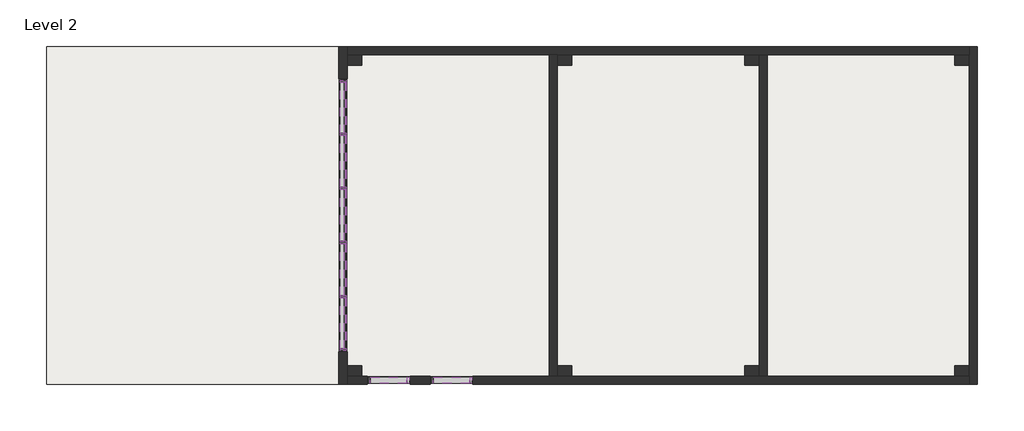
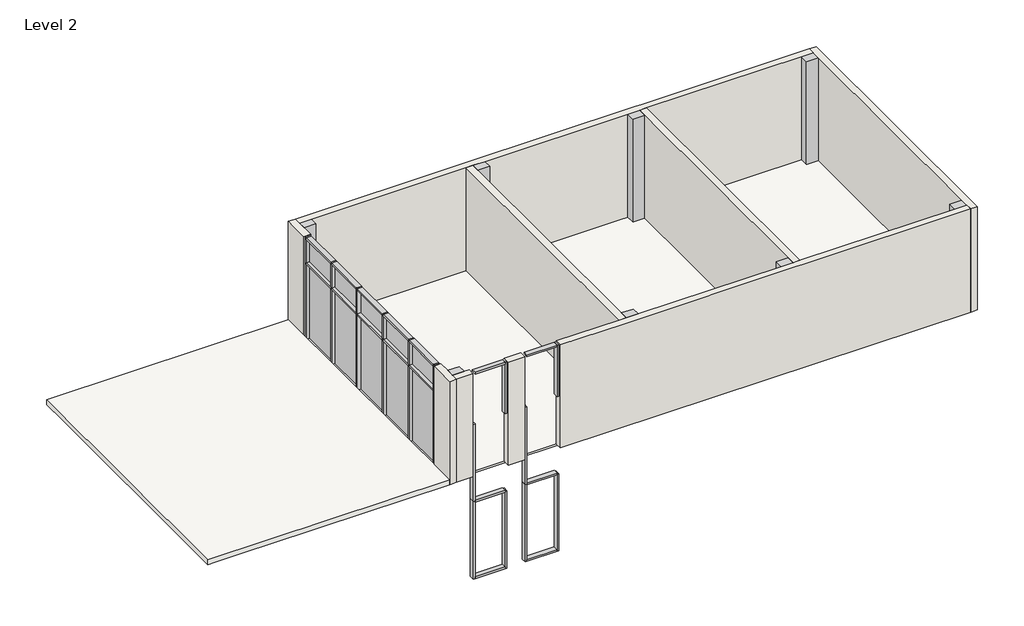
# One storey: 41 members, 10 plates, 9 walls, 8 columns, 3 slabs, 1 roof.
"""IFC4 building model written with IfcOpenShell, lengths in millimetres."""

import ifcopenshell
import ifcopenshell.guid

model = None  # the IFC model being written
_history = None  # IfcOwnerHistory: only IFC2X3 demands one
_inside = {}  # id of a spatial element -> (the spatial element, [elements in it])
_under = {}  # id of a project, library or spatial element -> (it, [spatial elements below it])
_declared = {}  # id of a project -> (the project, [libraries it declares])
_typed = {}  # id of a type object -> (the type object, [elements of that type])
_made_of = {}  # id of a material, layer set ... -> (it, [elements and type objects made of it])


def new_model(schema):
    """Start an empty IFC model of exactly this schema.

    Asked for "IFC4X3", IfcOpenShell would pick the latest addendum, in which some entities
    have other attributes; the version numbers below select the first issue.
    IFC2X3 requires an IfcOwnerHistory on every rooted entity: one is made here for all.
    """
    global model, _history
    if schema == "IFC4X3":
        model = ifcopenshell.file(schema_version=(4, 3, 0, 0))
    else:
        model = ifcopenshell.file(schema=schema)
    _inside.clear()
    _under.clear()
    _declared.clear()
    _typed.clear()
    _made_of.clear()
    _history = None
    if model.schema == "IFC2X3":
        org = make("IfcOrganization", Name="unknown")
        user = make(
            "IfcPersonAndOrganization",
            ThePerson=make("IfcPerson", FamilyName="unknown"),
            TheOrganization=org,
        )
        app = make(
            "IfcApplication",
            ApplicationDeveloper=org,
            Version="unknown",
            ApplicationFullName="unknown",
            ApplicationIdentifier="unknown",
        )
        _history = make(
            "IfcOwnerHistory",
            OwningUser=user,
            OwningApplication=app,
            ChangeAction="ADDED",
            CreationDate=0,
        )
    return model


def make(cls, **values):
    """One entity of the class cls with the attributes given. An attribute that is None is left unset."""
    return model.create_entity(
        cls, **{name: value for name, value in values.items() if value is not None}
    )


def rooted(cls, **values):
    """An entity with a GlobalId (a new one), such as an element, a storey or a relation."""
    return make(cls, GlobalId=ifcopenshell.guid.new(), OwnerHistory=_history, **values)


def si_unit(unit_type, name, prefix=None):
    """IfcSIUnit, for example si_unit("LENGTHUNIT", "METRE", prefix="MILLI")."""
    return make("IfcSIUnit", UnitType=unit_type, Prefix=prefix, Name=name)


def assignment(units):
    """IfcUnitAssignment: the units of a project."""
    return None if units is None else make("IfcUnitAssignment", Units=units)


def point(xyz):
    """IfcCartesianPoint."""
    return None if xyz is None else make("IfcCartesianPoint", Coordinates=xyz)


def direction(xyz):
    """IfcDirection."""
    return None if xyz is None else make("IfcDirection", DirectionRatios=xyz)


def frame(location, z_axis=None, x_axis=None):
    """IfcAxis2Placement3D, a coordinate frame: its origin and axes. An axis left out is left unset."""
    return make(
        "IfcAxis2Placement3D",
        Location=point(location),
        Axis=direction(z_axis),
        RefDirection=direction(x_axis),
    )


def origin():
    """The frame at (0, 0, 0) with its axes left unset."""
    return frame((0.0, 0.0, 0.0))


def origin_with_axes():
    """The frame at (0, 0, 0) with the z axis (0, 0, 1) and the x axis (1, 0, 0) written out."""
    return frame((0.0, 0.0, 0.0), z_axis=(0.0, 0.0, 1.0), x_axis=(1.0, 0.0, 0.0))


def place(relative_to, where):
    """IfcLocalPlacement: puts the frame where relative to a parent placement (None: the world)."""
    return make(
        "IfcLocalPlacement", PlacementRelTo=relative_to, RelativePlacement=where
    )


def context(
    kind, dimensions, precision=None, world=None, true_north=None, identifier=None
):
    """IfcGeometricRepresentationContext, for example the 3D "Model" context."""
    return make(
        "IfcGeometricRepresentationContext",
        ContextIdentifier=identifier,
        ContextType=kind,
        CoordinateSpaceDimension=dimensions,
        Precision=precision,
        WorldCoordinateSystem=world,
        TrueNorth=true_north,
    )


def project(units=None, contexts=None):
    """IfcProject with its units and contexts."""
    return rooted(
        "IfcProject",
        Name="project",
        RepresentationContexts=contexts,
        UnitsInContext=assignment(units),
    )


def spatial(cls, under=None, at=None, **own):
    """A site, building, storey or space (cls), placed at a placement, below another one or the project."""
    s = rooted(cls, ObjectPlacement=at, **own)
    if under is not None:
        _under.setdefault(under.id(), (under, []))[1].append(s)
    return s


def polyline(points):
    """IfcPolyline through the points."""
    return make("IfcPolyline", Points=[point(p) for p in points])


def outline(outer, holes=None, kind="AREA"):
    """IfcArbitraryClosedProfileDef: a profile drawn as a closed curve; with holes, ...WithVoids."""
    if holes is None:
        return make("IfcArbitraryClosedProfileDef", ProfileType=kind, OuterCurve=outer)
    return make(
        "IfcArbitraryProfileDefWithVoids",
        ProfileType=kind,
        OuterCurve=outer,
        InnerCurves=holes,
    )


def extrude(swept, where, along, depth):
    """IfcExtrudedAreaSolid: the profile swept, set in the frame where, extruded along a direction by depth."""
    return make(
        "IfcExtrudedAreaSolid",
        SweptArea=swept,
        Position=where,
        ExtrudedDirection=direction(along),
        Depth=depth,
    )


def faces_of(points, faces, orient=None, outer=None):
    """IfcFace entities. A face is a list of loops; a loop is a list of indices into points, from 0.

    orient and outer hold one flag for each loop. By default every Orientation is true, the
    first loop of a face is its IfcFaceOuterBound and the others are IfcFaceBound.
    """
    made = []
    for i, loops in enumerate(faces):
        bounds = []
        for j, loop in enumerate(loops):
            is_outer = j == 0 if outer is None else outer[i][j]
            bounds.append(
                make(
                    "IfcFaceOuterBound" if is_outer else "IfcFaceBound",
                    Bound=make("IfcPolyLoop", Polygon=[points[k] for k in loop]),
                    Orientation=True if orient is None else orient[i][j],
                )
            )
        made.append(make("IfcFace", Bounds=bounds))
    return made


def faceted_brep(points, faces, orient=None, outer=None, voids=None):
    """IfcFacetedBrep: a solid bounded by flat faces; with voids (closed shells), ...WithVoids."""
    shared = [point(p) for p in points]
    hull = make("IfcClosedShell", CfsFaces=faces_of(shared, faces, orient, outer))
    if voids is None:
        return make("IfcFacetedBrep", Outer=hull)
    return make(
        "IfcFacetedBrepWithVoids",
        Outer=hull,
        Voids=[
            make(cls, CfsFaces=faces_of(shared, fs, o, b)) for cls, fs, o, b in voids
        ],
    )


def shape(context_of_items, identifier, shape_type, items):
    """IfcShapeRepresentation: the items that make up one representation, for example the "Body"."""
    return make(
        "IfcShapeRepresentation",
        ContextOfItems=context_of_items,
        RepresentationIdentifier=identifier,
        RepresentationType=shape_type,
        Items=items,
    )


def source(mapping_origin, context_of_items, identifier, shape_type, items):
    """IfcRepresentationMap: a shape defined once, which mapped items show again and again."""
    return make(
        "IfcRepresentationMap",
        MappingOrigin=mapping_origin,
        MappedRepresentation=shape(context_of_items, identifier, shape_type, items),
    )


def transform(
    local_origin,
    x_axis=None,
    y_axis=None,
    z_axis=None,
    scale=None,
    scale2=None,
    scale3=None,
    uniform=True,
):
    """IfcCartesianTransformationOperator3D, or its non-uniform kind. x_axis, y_axis, z_axis: its Axis1, 2, 3."""
    if uniform:
        return make(
            "IfcCartesianTransformationOperator3D",
            Axis1=direction(x_axis),
            Axis2=direction(y_axis),
            LocalOrigin=point(local_origin),
            Scale=scale,
            Axis3=direction(z_axis),
        )
    return make(
        "IfcCartesianTransformationOperator3DnonUniform",
        Axis1=direction(x_axis),
        Axis2=direction(y_axis),
        LocalOrigin=point(local_origin),
        Scale=scale,
        Axis3=direction(z_axis),
        Scale2=scale2,
        Scale3=scale3,
    )


def mapped(mapping_source, mapping_target):
    """IfcMappedItem: shows the shape of a source again, moved by a transform."""
    return make(
        "IfcMappedItem", MappingSource=mapping_source, MappingTarget=mapping_target
    )


def made_of(thing, what):
    """Note that an element or type object is made of a material, layer set ...; save() writes the relation."""
    if what is not None:
        _made_of.setdefault(what.id(), (what, []))[1].append(thing)
    return thing


def element(
    cls,
    number,
    at=None,
    inside=None,
    cuts=None,
    type_object=None,
    material=None,
    context=None,
    identifier="Body",
    shape_type=None,
    held_by="IfcProductDefinitionShape",
    body=None,
    shapes=None,
    **own,
):
    """One element of the class cls, such as IfcWall. Its Tag is "e" and its number.

    at: its placement. inside: the storey or other place that contains it. cuts: it is an
    opening in that element (IfcRelVoidsElement). A single representation is given by context,
    identifier, shape_type and body (its items); several are given by shapes. held_by: the class
    of the entity that holds the representations. save() writes the other relations.
    """
    e = rooted(cls, Tag="e%d" % number, ObjectPlacement=at, **own)
    if body is not None:
        shapes = [shape(context, identifier, shape_type, body)]
    if shapes is not None:
        e.Representation = make(held_by, Representations=shapes)
    if inside is not None:
        _inside.setdefault(inside.id(), (inside, []))[1].append(e)
    if cuts is not None:
        rooted(
            "IfcRelVoidsElement", RelatingBuildingElement=cuts, RelatedOpeningElement=e
        )
    if type_object is not None:
        _typed.setdefault(type_object.id(), (type_object, []))[1].append(e)
    return made_of(e, material)


def aggregate(whole, parts):
    """IfcRelAggregates: a whole, such as a stair, and the parts it consists of."""
    return rooted("IfcRelAggregates", RelatingObject=whole, RelatedObjects=parts)


def save(model, path):
    """Write the relations noted so far, then the file.

    IfcRelAggregates (storeys below a building ...), IfcRelContainedInSpatialStructure (elements
    in a storey), IfcRelDefinesByType, IfcRelAssociatesMaterial and IfcRelDeclares: one each for
    every whole, place, type object, material and project.
    """
    for whole, parts in _under.values():
        aggregate(whole, parts)
    for where, things in _inside.values():
        rooted(
            "IfcRelContainedInSpatialStructure",
            RelatedElements=things,
            RelatingStructure=where,
        )
    for kind, things in _typed.values():
        rooted("IfcRelDefinesByType", RelatedObjects=things, RelatingType=kind)
    for what, things in _made_of.values():
        rooted("IfcRelAssociatesMaterial", RelatedObjects=things, RelatingMaterial=what)
    for by, libraries in _declared.values():
        rooted("IfcRelDeclares", RelatingContext=by, RelatedDefinitions=libraries)
    model.write(path)


def rectangular_mullion_50_x_150mm_49395e3f(model_context):
    return source(origin(), model_context, "Body", "SweptSolid", [
        extrude(outline(polyline([(0.0, 75.0), (0.0, -75.0), (-50.0, -75.0), (-50.0, 75.0), (0.0, 75.0)])), frame((0.0, 0.0, -1240.0000002), z_axis=(0.0, 0.0, 1.0), x_axis=(1.0, 0.0, 0.0)), (0.0, 0.0, 1.0), 1240.0000002),
    ])


def rectangular_mullion_50_x_150mm_673792d4(model_context):
    return source(origin(), model_context, "Body", "SweptSolid", [
        extrude(outline(polyline([(0.0, 75.0), (0.0, -75.0), (-50.0, -75.0), (-50.0, 75.0), (0.0, 75.0)])), frame((0.0, 0.0, -1264.9999999), z_axis=(0.0, 0.0, 1.0), x_axis=(1.0, 0.0, 0.0)), (0.0, 0.0, 1.0), 1264.9999999),
    ])


def rectangular_mullion_50_x_150mm_23e890aa(model_context):
    return source(origin(), model_context, "Body", "SweptSolid", [
        extrude(outline(polyline([(25.0, 75.0), (25.0, -75.0), (-25.0, -75.0), (-25.0, 75.0), (25.0, 75.0)])), frame((0.0, 0.0, -1240.0000002), z_axis=(0.0, 0.0, 1.0), x_axis=(1.0, 0.0, 0.0)), (0.0, 0.0, 1.0), 1240.0000002),
    ])


def rectangular_mullion_50_x_150mm_97c2790d(model_context):
    return source(origin(), model_context, "Body", "SweptSolid", [
        extrude(outline(polyline([(25.0, 75.0), (25.0, -75.0), (-25.0, -75.0), (-25.0, 75.0), (25.0, 75.0)])), frame((0.0, 0.0, -1264.9999999), z_axis=(0.0, 0.0, 1.0), x_axis=(1.0, 0.0, 0.0)), (0.0, 0.0, 1.0), 1264.9999999),
    ])


def rectangular_mullion_50_x_150mm_6225e4e3(model_context):
    return source(origin(), model_context, "Body", "SweptSolid", [
        extrude(outline(polyline([(25.0, 75.0), (25.0, -75.0), (-25.0, -75.0), (-25.0, 75.0), (25.0, 75.0)])), frame((0.0, 0.0, -2400.0), z_axis=(0.0, 0.0, 1.0), x_axis=(1.0, 0.0, 0.0)), (0.0, 0.0, 1.0), 2400.0),
    ])


def rectangular_mullion_50_x_150mm_14f10ac7(model_context):
    return source(origin(), model_context, "Body", "SweptSolid", [
        extrude(outline(polyline([(25.0, 75.0), (25.0, -75.0), (-25.0, -75.0), (-25.0, 75.0), (25.0, 75.0)])), frame((0.0, 0.0, -800.0), z_axis=(0.0, 0.0, 1.0), x_axis=(1.0, 0.0, 0.0)), (0.0, 0.0, 1.0), 800.0),
    ])


def rectangular_mullion_50_x_150mm_662c37b1(model_context):
    return source(origin(), model_context, "Body", "SweptSolid", [
        extrude(outline(polyline([(0.0, 75.0), (0.0, -75.0), (-50.0, -75.0), (-50.0, 75.0), (0.0, 75.0)])), frame((0.0, 0.0, -2400.0), z_axis=(0.0, 0.0, 1.0), x_axis=(1.0, 0.0, 0.0)), (0.0, 0.0, 1.0), 2400.0),
    ])


def rectangular_mullion_50_x_150mm_6ffebc0f(model_context):
    return source(origin(), model_context, "Body", "SweptSolid", [
        extrude(outline(polyline([(0.0, 75.0), (0.0, -75.0), (-50.0, -75.0), (-50.0, 75.0), (0.0, 75.0)])), frame((0.0, 0.0, -800.0), z_axis=(0.0, 0.0, 1.0), x_axis=(1.0, 0.0, 0.0)), (0.0, 0.0, 1.0), 800.0),
    ])


def rectangular_mullion_50_x_150mm_8ee200a5(model_context):
    return source(origin(), model_context, "Body", "SweptSolid", [
        extrude(outline(polyline([(0.0, 75.0), (0.0, -75.0), (-50.0, -75.0), (-50.0, 75.0), (0.0, 75.0)])), frame((0.0, 0.0, -887.5), z_axis=(0.0, 0.0, 1.0), x_axis=(1.0, 0.0, 0.0)), (0.0, 0.0, 1.0), 887.5),
    ])


def rectangular_mullion_50_x_150mm_6e645c27(model_context):
    return source(origin(), model_context, "Body", "SweptSolid", [
        extrude(outline(polyline([(25.0, 75.0), (25.0, -75.0), (-25.0, -75.0), (-25.0, 75.0), (25.0, 75.0)])), frame((0.0, 0.0, -887.5), z_axis=(0.0, 0.0, 1.0), x_axis=(1.0, 0.0, 0.0)), (0.0, 0.0, 1.0), 887.5),
    ])


def rectangular_mullion_50_x_150mm_849620c7(model_context):
    return source(origin(), model_context, "Body", "SweptSolid", [
        extrude(outline(polyline([(0.0, 75.0), (0.0, -75.0), (-50.0, -75.0), (-50.0, 75.0), (0.0, 75.0)])), frame((0.0, 0.0, -1600.0), z_axis=(0.0, 0.0, 1.0), x_axis=(1.0, 0.0, 0.0)), (0.0, 0.0, 1.0), 1600.0),
    ])


def system_panel_glazed_da598795(model_context):
    return source(origin(), model_context, "Body", "SweptSolid", [
        extrude(outline(polyline([(620.0000001, 24.5), (-620.0000001, 24.5), (-620.0000001, 49.5), (620.0000001, 49.5), (620.0000001, 24.5)])), origin_with_axes(), (0.0, 0.0, 1.0), 2325.0),
    ])


def system_panel_glazed_e4649fa4(model_context):
    return source(origin(), model_context, "Body", "SweptSolid", [
        extrude(outline(polyline([(632.4999999, 24.5), (-632.4999999, 24.5), (-632.4999999, 49.5), (632.4999999, 49.5), (632.4999999, 24.5)])), origin_with_axes(), (0.0, 0.0, 1.0), 2325.0),
    ])


def system_panel_glazed_8692f37a(model_context):
    return source(origin(), model_context, "Body", "SweptSolid", [
        extrude(outline(polyline([(620.0000001, 24.5), (-620.0000001, 24.5), (-620.0000001, 49.5), (620.0000001, 49.5), (620.0000001, 24.5)])), origin_with_axes(), (0.0, 0.0, 1.0), 725.0),
    ])


def system_panel_glazed_8e5047c4(model_context):
    return source(origin(), model_context, "Body", "SweptSolid", [
        extrude(outline(polyline([(632.4999999, 24.5), (-632.4999999, 24.5), (-632.4999999, 49.5), (632.4999999, 49.5), (632.4999999, 24.5)])), origin_with_axes(), (0.0, 0.0, 1.0), 725.0),
    ])


model = new_model("IFC4")

# Units and contexts
model_context = context("Model", 3, world=origin())
ifc_project = project(units=[si_unit("LENGTHUNIT", "METRE", prefix="MILLI")], contexts=[model_context])

# Site, building, storey
site = spatial("IfcSite", under=ifc_project)
building = spatial("IfcBuilding", under=site)
storey = spatial("IfcBuildingStorey", under=building, Name="Level 2", Elevation=3200.0)

# Columns
placement = place(None, origin())
element("IfcColumn", 1, ObjectType="M_Rectangular Column : 350 X 250", at=placement, inside=storey, context=model_context, shape_type="SweptSolid", body=[
    extrude(outline(polyline([(4723.8381324, 10606.2894154), (5073.8381324, 10606.2894154), (5073.8381324, 10356.2894154), (4723.8381324, 10356.2894154), (4723.8381324, 10606.2894154)])), frame((0.0, 0.0, 3200.0), z_axis=(0.0, 0.0, 1.0), x_axis=(1.0, 0.0, 0.0)), (0.0, 0.0, 1.0), 3200.0),
])
element("IfcColumn", 2, ObjectType="M_Rectangular Column : 350 X 250", at=placement, inside=storey, context=model_context, shape_type="SweptSolid", body=[
    extrude(outline(polyline([(4723.8381324, 3056.2894154), (5073.8381324, 3056.2894154), (5073.8381324, 2806.2894154), (4723.8381324, 2806.2894154), (4723.8381324, 3056.2894154)])), frame((0.0, 0.0, 3200.0), z_axis=(0.0, 0.0, 1.0), x_axis=(1.0, 0.0, 0.0)), (0.0, 0.0, 1.0), 3200.0),
])
element("IfcColumn", 3, ObjectType="M_Rectangular Column : 350 X 250", at=placement, inside=storey, context=model_context, shape_type="SweptSolid", body=[
    extrude(outline(polyline([(-376.1618676, 3056.2894154), (-26.1618676, 3056.2894154), (-26.1618676, 2806.2894154), (-376.1618676, 2806.2894154), (-376.1618676, 3056.2894154)])), frame((0.0, 0.0, 3200.0), z_axis=(0.0, 0.0, 1.0), x_axis=(1.0, 0.0, 0.0)), (0.0, 0.0, 1.0), 3200.0),
])
element("IfcColumn", 4, ObjectType="M_Rectangular Column : 350 X 250", at=placement, inside=storey, context=model_context, shape_type="SweptSolid", body=[
    extrude(outline(polyline([(-376.1618676, 10606.2894154), (-26.1618676, 10606.2894154), (-26.1618676, 10356.2894154), (-376.1618676, 10356.2894154), (-376.1618676, 10606.2894154)])), frame((0.0, 0.0, 3200.0), z_axis=(0.0, 0.0, 1.0), x_axis=(1.0, 0.0, 0.0)), (0.0, 0.0, 1.0), 3200.0),
])
element("IfcColumn", 5, ObjectType="M_Rectangular Column : 350 X 250", at=placement, inside=storey, context=model_context, shape_type="SweptSolid", body=[
    extrude(outline(polyline([(-4926.1618676, 10606.2894154), (-4576.1618676, 10606.2894154), (-4576.1618676, 10356.2894154), (-4926.1618676, 10356.2894154), (-4926.1618676, 10606.2894154)])), frame((0.0, 0.0, 3200.0), z_axis=(0.0, 0.0, 1.0), x_axis=(1.0, 0.0, 0.0)), (0.0, 0.0, 1.0), 3200.0),
])
element("IfcColumn", 6, ObjectType="M_Rectangular Column : 350 X 250", at=placement, inside=storey, context=model_context, shape_type="SweptSolid", body=[
    extrude(outline(polyline([(-4926.1618676, 3056.2894154), (-4576.1618676, 3056.2894154), (-4576.1618676, 2806.2894154), (-4926.1618676, 2806.2894154), (-4926.1618676, 3056.2894154)])), frame((0.0, 0.0, 3200.0), z_axis=(0.0, 0.0, 1.0), x_axis=(1.0, 0.0, 0.0)), (0.0, 0.0, 1.0), 3200.0),
])
element("IfcColumn", 7, ObjectType="M_Rectangular Column : 350 X 250", at=placement, inside=storey, context=model_context, shape_type="SweptSolid", body=[
    extrude(outline(polyline([(-10026.1618676, 3056.2894154), (-9676.1618676, 3056.2894154), (-9676.1618676, 2806.2894154), (-10026.1618676, 2806.2894154), (-10026.1618676, 3056.2894154)])), frame((0.0, 0.0, 3200.0), z_axis=(0.0, 0.0, 1.0), x_axis=(1.0, 0.0, 0.0)), (0.0, 0.0, 1.0), 3200.0),
])
element("IfcColumn", 8, ObjectType="M_Rectangular Column : 350 X 250", at=placement, inside=storey, context=model_context, shape_type="SweptSolid", body=[
    extrude(outline(polyline([(-10026.1618676, 10606.2894154), (-9676.1618676, 10606.2894154), (-9676.1618676, 10356.2894154), (-10026.1618676, 10356.2894154), (-10026.1618676, 10606.2894154)])), frame((0.0, 0.0, 3200.0), z_axis=(0.0, 0.0, 1.0), x_axis=(1.0, 0.0, 0.0)), (0.0, 0.0, 1.0), 3200.0),
])

# Members
rectangular_mullion_50_x_150mm_shape = rectangular_mullion_50_x_150mm_49395e3f(model_context)
element("IfcMember", 9, ObjectType="Rectangular Mullion : 50 x 150mm", at=placement, inside=storey, context=model_context, shape_type="MappedRepresentation", body=[
    mapped(rectangular_mullion_50_x_150mm_shape, transform((-10126.1618676, 3468.7894154, 6400.0), x_axis=(0.0, 0.0, 1.0), y_axis=(-1.0, 0.0, 0.0), z_axis=(0.0, -1.0, 0.0))),
])
element("IfcMember", 10, ObjectType="Rectangular Mullion : 50 x 150mm", at=placement, inside=storey, context=model_context, shape_type="MappedRepresentation", body=[
    mapped(rectangular_mullion_50_x_150mm_shape, transform((-10126.1618676, 8703.7894152, 6400.0), x_axis=(0.0, 0.0, 1.0), y_axis=(-1.0, 0.0, 0.0), z_axis=(0.0, -1.0, 0.0))),
])
element("IfcMember", 11, ObjectType="Rectangular Mullion : 50 x 150mm", at=placement, inside=storey, context=model_context, shape_type="MappedRepresentation", body=[
    mapped(rectangular_mullion_50_x_150mm_shape, transform((-10126.1618676, 9943.7894154, 3200.0), x_axis=(0.0, 0.0, -1.0), y_axis=(-1.0, 0.0, 0.0), z_axis=(0.0, 1.0, 0.0))),
])
element("IfcMember", 12, ObjectType="Rectangular Mullion : 50 x 150mm", at=placement, inside=storey, context=model_context, shape_type="MappedRepresentation", body=[
    mapped(rectangular_mullion_50_x_150mm_shape, transform((-10126.1618676, 4708.7894156, 3200.0), x_axis=(0.0, 0.0, -1.0), y_axis=(-1.0, 0.0, 0.0), z_axis=(0.0, 1.0, 0.0))),
])
rectangular_mullion_50_x_150mm_2_shape = rectangular_mullion_50_x_150mm_673792d4(model_context)
element("IfcMember", 13, ObjectType="Rectangular Mullion : 50 x 150mm", at=placement, inside=storey, context=model_context, shape_type="MappedRepresentation", body=[
    mapped(rectangular_mullion_50_x_150mm_2_shape, transform((-10126.1618676, 7388.7894153, 6400.0), x_axis=(0.0, 0.0, 1.0), y_axis=(-1.0, 0.0, 0.0), z_axis=(0.0, -1.0, 0.0))),
])
element("IfcMember", 14, ObjectType="Rectangular Mullion : 50 x 150mm", at=placement, inside=storey, context=model_context, shape_type="MappedRepresentation", body=[
    mapped(rectangular_mullion_50_x_150mm_2_shape, transform((-10126.1618676, 6073.7894154, 6400.0), x_axis=(0.0, 0.0, 1.0), y_axis=(-1.0, 0.0, 0.0), z_axis=(0.0, -1.0, 0.0))),
])
element("IfcMember", 15, ObjectType="Rectangular Mullion : 50 x 150mm", at=placement, inside=storey, context=model_context, shape_type="MappedRepresentation", body=[
    mapped(rectangular_mullion_50_x_150mm_2_shape, transform((-10126.1618676, 4758.7894156, 6400.0), x_axis=(0.0, 0.0, 1.0), y_axis=(-1.0, 0.0, 0.0), z_axis=(0.0, -1.0, 0.0))),
])
element("IfcMember", 16, ObjectType="Rectangular Mullion : 50 x 150mm", at=placement, inside=storey, context=model_context, shape_type="MappedRepresentation", body=[
    mapped(rectangular_mullion_50_x_150mm_2_shape, transform((-10126.1618676, 8653.7894152, 3200.0), x_axis=(0.0, 0.0, -1.0), y_axis=(-1.0, 0.0, 0.0), z_axis=(0.0, 1.0, 0.0))),
])
element("IfcMember", 17, ObjectType="Rectangular Mullion : 50 x 150mm", at=placement, inside=storey, context=model_context, shape_type="MappedRepresentation", body=[
    mapped(rectangular_mullion_50_x_150mm_2_shape, transform((-10126.1618676, 7338.7894153, 3200.0), x_axis=(0.0, 0.0, -1.0), y_axis=(-1.0, 0.0, 0.0), z_axis=(0.0, 1.0, 0.0))),
])
element("IfcMember", 18, ObjectType="Rectangular Mullion : 50 x 150mm", at=placement, inside=storey, context=model_context, shape_type="MappedRepresentation", body=[
    mapped(rectangular_mullion_50_x_150mm_2_shape, transform((-10126.1618676, 6023.7894154, 3200.0), x_axis=(0.0, 0.0, -1.0), y_axis=(-1.0, 0.0, 0.0), z_axis=(0.0, 1.0, 0.0))),
])
rectangular_mullion_50_x_150mm_3_shape = rectangular_mullion_50_x_150mm_23e890aa(model_context)
element("IfcMember", 19, ObjectType="Rectangular Mullion : 50 x 150mm", at=placement, inside=storey, context=model_context, shape_type="MappedRepresentation", body=[
    mapped(rectangular_mullion_50_x_150mm_3_shape, transform((-10126.1618676, 8703.7894152, 5600.0), x_axis=(0.0, 0.0, 1.0), y_axis=(-1.0, 0.0, 0.0), z_axis=(0.0, -1.0, 0.0))),
])
element("IfcMember", 20, ObjectType="Rectangular Mullion : 50 x 150mm", at=placement, inside=storey, context=model_context, shape_type="MappedRepresentation", body=[
    mapped(rectangular_mullion_50_x_150mm_3_shape, transform((-10126.1618676, 3468.7894154, 5600.0), x_axis=(0.0, 0.0, 1.0), y_axis=(-1.0, 0.0, 0.0), z_axis=(0.0, -1.0, 0.0))),
])
rectangular_mullion_50_x_150mm_4_shape = rectangular_mullion_50_x_150mm_97c2790d(model_context)
element("IfcMember", 21, ObjectType="Rectangular Mullion : 50 x 150mm", at=placement, inside=storey, context=model_context, shape_type="MappedRepresentation", body=[
    mapped(rectangular_mullion_50_x_150mm_4_shape, transform((-10126.1618676, 7388.7894153, 5600.0), x_axis=(0.0, 0.0, 1.0), y_axis=(-1.0, 0.0, 0.0), z_axis=(0.0, -1.0, 0.0))),
])
element("IfcMember", 22, ObjectType="Rectangular Mullion : 50 x 150mm", at=placement, inside=storey, context=model_context, shape_type="MappedRepresentation", body=[
    mapped(rectangular_mullion_50_x_150mm_4_shape, transform((-10126.1618676, 6073.7894154, 5600.0), x_axis=(0.0, 0.0, 1.0), y_axis=(-1.0, 0.0, 0.0), z_axis=(0.0, -1.0, 0.0))),
])
element("IfcMember", 23, ObjectType="Rectangular Mullion : 50 x 150mm", at=placement, inside=storey, context=model_context, shape_type="MappedRepresentation", body=[
    mapped(rectangular_mullion_50_x_150mm_4_shape, transform((-10126.1618676, 4758.7894156, 5600.0), x_axis=(0.0, 0.0, 1.0), y_axis=(-1.0, 0.0, 0.0), z_axis=(0.0, -1.0, 0.0))),
])
rectangular_mullion_50_x_150mm_5_shape = rectangular_mullion_50_x_150mm_6225e4e3(model_context)
element("IfcMember", 24, ObjectType="Rectangular Mullion : 50 x 150mm", at=placement, inside=storey, context=model_context, shape_type="MappedRepresentation", body=[
    mapped(rectangular_mullion_50_x_150mm_5_shape, transform((-10126.1618676, 8678.7894152, 3200.0), x_axis=(0.0, -1.0, 0.0), y_axis=(-1.0, 0.0, 0.0), z_axis=(0.0, 0.0, -1.0))),
])
element("IfcMember", 25, ObjectType="Rectangular Mullion : 50 x 150mm", at=placement, inside=storey, context=model_context, shape_type="MappedRepresentation", body=[
    mapped(rectangular_mullion_50_x_150mm_5_shape, transform((-10126.1618676, 7363.7894153, 3200.0), x_axis=(0.0, -1.0, 0.0), y_axis=(-1.0, 0.0, 0.0), z_axis=(0.0, 0.0, -1.0))),
])
element("IfcMember", 26, ObjectType="Rectangular Mullion : 50 x 150mm", at=placement, inside=storey, context=model_context, shape_type="MappedRepresentation", body=[
    mapped(rectangular_mullion_50_x_150mm_5_shape, transform((-10126.1618676, 6048.7894154, 3200.0), x_axis=(0.0, -1.0, 0.0), y_axis=(-1.0, 0.0, 0.0), z_axis=(0.0, 0.0, -1.0))),
])
element("IfcMember", 27, ObjectType="Rectangular Mullion : 50 x 150mm", at=placement, inside=storey, context=model_context, shape_type="MappedRepresentation", body=[
    mapped(rectangular_mullion_50_x_150mm_5_shape, transform((-10126.1618676, 4733.7894156, 3200.0), x_axis=(0.0, -1.0, 0.0), y_axis=(-1.0, 0.0, 0.0), z_axis=(0.0, 0.0, -1.0))),
])
rectangular_mullion_50_x_150mm_6_shape = rectangular_mullion_50_x_150mm_14f10ac7(model_context)
element("IfcMember", 28, ObjectType="Rectangular Mullion : 50 x 150mm", at=placement, inside=storey, context=model_context, shape_type="MappedRepresentation", body=[
    mapped(rectangular_mullion_50_x_150mm_6_shape, transform((-10126.1618676, 8678.7894152, 5600.0), x_axis=(0.0, -1.0, 0.0), y_axis=(-1.0, 0.0, 0.0), z_axis=(0.0, 0.0, -1.0))),
])
element("IfcMember", 29, ObjectType="Rectangular Mullion : 50 x 150mm", at=placement, inside=storey, context=model_context, shape_type="MappedRepresentation", body=[
    mapped(rectangular_mullion_50_x_150mm_6_shape, transform((-10126.1618676, 7363.7894153, 5600.0), x_axis=(0.0, -1.0, 0.0), y_axis=(-1.0, 0.0, 0.0), z_axis=(0.0, 0.0, -1.0))),
])
element("IfcMember", 30, ObjectType="Rectangular Mullion : 50 x 150mm", at=placement, inside=storey, context=model_context, shape_type="MappedRepresentation", body=[
    mapped(rectangular_mullion_50_x_150mm_6_shape, transform((-10126.1618676, 6048.7894154, 5600.0), x_axis=(0.0, -1.0, 0.0), y_axis=(-1.0, 0.0, 0.0), z_axis=(0.0, 0.0, -1.0))),
])
element("IfcMember", 31, ObjectType="Rectangular Mullion : 50 x 150mm", at=placement, inside=storey, context=model_context, shape_type="MappedRepresentation", body=[
    mapped(rectangular_mullion_50_x_150mm_6_shape, transform((-10126.1618676, 4733.7894156, 5600.0), x_axis=(0.0, -1.0, 0.0), y_axis=(-1.0, 0.0, 0.0), z_axis=(0.0, 0.0, -1.0))),
])
rectangular_mullion_50_x_150mm_7_shape = rectangular_mullion_50_x_150mm_662c37b1(model_context)
element("IfcMember", 32, ObjectType="Rectangular Mullion : 50 x 150mm", at=placement, inside=storey, context=model_context, shape_type="MappedRepresentation", body=[
    mapped(rectangular_mullion_50_x_150mm_7_shape, transform((-10126.1618676, 3418.7894154, 3200.0), x_axis=(0.0, -1.0, 0.0), y_axis=(-1.0, 0.0, 0.0), z_axis=(0.0, 0.0, -1.0))),
])
element("IfcMember", 33, ObjectType="Rectangular Mullion : 50 x 150mm", at=placement, inside=storey, context=model_context, shape_type="MappedRepresentation", body=[
    mapped(rectangular_mullion_50_x_150mm_7_shape, transform((-9513.6618676, 2706.2894154, 0.0), x_axis=(-1.0, 0.0, 0.0), y_axis=(0.0, 1.0, 0.0), z_axis=(0.0, 0.0, -1.0))),
])
element("IfcMember", 34, ObjectType="Rectangular Mullion : 50 x 150mm", at=placement, inside=storey, context=model_context, shape_type="MappedRepresentation", body=[
    mapped(rectangular_mullion_50_x_150mm_7_shape, transform((-7988.6618676, 2706.2894154, 0.0), x_axis=(-1.0, 0.0, 0.0), y_axis=(0.0, 1.0, 0.0), z_axis=(0.0, 0.0, -1.0))),
])
rectangular_mullion_50_x_150mm_8_shape = rectangular_mullion_50_x_150mm_6ffebc0f(model_context)
element("IfcMember", 35, ObjectType="Rectangular Mullion : 50 x 150mm", at=placement, inside=storey, context=model_context, shape_type="MappedRepresentation", body=[
    mapped(rectangular_mullion_50_x_150mm_8_shape, transform((-10126.1618676, 9993.7894154, 6400.0), x_axis=(0.0, 1.0, 0.0), y_axis=(-1.0, 0.0, 0.0), z_axis=(0.0, 0.0, 1.0))),
])
element("IfcMember", 36, ObjectType="Rectangular Mullion : 50 x 150mm", at=placement, inside=storey, context=model_context, shape_type="MappedRepresentation", body=[
    mapped(rectangular_mullion_50_x_150mm_8_shape, transform((-10126.1618676, 3418.7894154, 5600.0), x_axis=(0.0, -1.0, 0.0), y_axis=(-1.0, 0.0, 0.0), z_axis=(0.0, 0.0, -1.0))),
])
element("IfcMember", 37, ObjectType="Rectangular Mullion : 50 x 150mm", at=placement, inside=storey, context=model_context, shape_type="MappedRepresentation", body=[
    mapped(rectangular_mullion_50_x_150mm_7_shape, transform((-10126.1618676, 9993.7894154, 5600.0), x_axis=(0.0, 1.0, 0.0), y_axis=(-1.0, 0.0, 0.0), z_axis=(0.0, 0.0, 1.0))),
])
element("IfcMember", 38, ObjectType="Rectangular Mullion : 50 x 150mm", at=placement, inside=storey, context=model_context, shape_type="MappedRepresentation", body=[
    mapped(rectangular_mullion_50_x_150mm_7_shape, transform((-8526.1618676, 2706.2894154, 2400.0), x_axis=(1.0, 0.0, 0.0), y_axis=(0.0, 1.0, 0.0), z_axis=(0.0, 0.0, 1.0))),
])
element("IfcMember", 39, ObjectType="Rectangular Mullion : 50 x 150mm", at=placement, inside=storey, context=model_context, shape_type="MappedRepresentation", body=[
    mapped(rectangular_mullion_50_x_150mm_7_shape, transform((-7001.1618676, 2706.2894154, 2400.0), x_axis=(1.0, 0.0, 0.0), y_axis=(0.0, 1.0, 0.0), z_axis=(0.0, 0.0, 1.0))),
])
rectangular_mullion_50_x_150mm_9_shape = rectangular_mullion_50_x_150mm_8ee200a5(model_context)
element("IfcMember", 40, ObjectType="Rectangular Mullion : 50 x 150mm", at=placement, inside=storey, context=model_context, shape_type="MappedRepresentation", body=[
    mapped(rectangular_mullion_50_x_150mm_9_shape, transform((-9463.6618676, 2706.2894154, 6400.0), x_axis=(0.0, 0.0, 1.0), y_axis=(0.0, 1.0, 0.0), z_axis=(-1.0, 0.0, 0.0))),
])
element("IfcMember", 41, ObjectType="Rectangular Mullion : 50 x 150mm", at=placement, inside=storey, context=model_context, shape_type="MappedRepresentation", body=[
    mapped(rectangular_mullion_50_x_150mm_9_shape, transform((-7938.6618676, 2706.2894154, 6400.0), x_axis=(0.0, 0.0, 1.0), y_axis=(0.0, 1.0, 0.0), z_axis=(-1.0, 0.0, 0.0))),
])
element("IfcMember", 42, ObjectType="Rectangular Mullion : 50 x 150mm", at=placement, inside=storey, context=model_context, shape_type="MappedRepresentation", body=[
    mapped(rectangular_mullion_50_x_150mm_9_shape, transform((-8576.1618676, 2706.2894154, 0.0), x_axis=(0.0, 0.0, -1.0), y_axis=(0.0, 1.0, 0.0), z_axis=(1.0, 0.0, 0.0))),
])
element("IfcMember", 43, ObjectType="Rectangular Mullion : 50 x 150mm", at=placement, inside=storey, context=model_context, shape_type="MappedRepresentation", body=[
    mapped(rectangular_mullion_50_x_150mm_9_shape, transform((-7051.1618676, 2706.2894154, 0.0), x_axis=(0.0, 0.0, -1.0), y_axis=(0.0, 1.0, 0.0), z_axis=(1.0, 0.0, 0.0))),
])
rectangular_mullion_50_x_150mm_10_shape = rectangular_mullion_50_x_150mm_6e645c27(model_context)
element("IfcMember", 44, ObjectType="Rectangular Mullion : 50 x 150mm", at=placement, inside=storey, context=model_context, shape_type="MappedRepresentation", body=[
    mapped(rectangular_mullion_50_x_150mm_10_shape, transform((-9463.6618676, 2706.2894154, 2400.0), x_axis=(0.0, 0.0, 1.0), y_axis=(0.0, 1.0, 0.0), z_axis=(-1.0, 0.0, 0.0))),
])
element("IfcMember", 45, ObjectType="Rectangular Mullion : 50 x 150mm", at=placement, inside=storey, context=model_context, shape_type="MappedRepresentation", body=[
    mapped(rectangular_mullion_50_x_150mm_10_shape, transform((-7938.6618676, 2706.2894154, 2400.0), x_axis=(0.0, 0.0, 1.0), y_axis=(0.0, 1.0, 0.0), z_axis=(-1.0, 0.0, 0.0))),
])
rectangular_mullion_50_x_150mm_11_shape = rectangular_mullion_50_x_150mm_849620c7(model_context)
element("IfcMember", 46, ObjectType="Rectangular Mullion : 50 x 150mm", at=placement, inside=storey, context=model_context, shape_type="MappedRepresentation", body=[
    mapped(rectangular_mullion_50_x_150mm_11_shape, transform((-8526.1618676, 2706.2894154, 6400.0), x_axis=(1.0, 0.0, 0.0), y_axis=(0.0, 1.0, 0.0), z_axis=(0.0, 0.0, 1.0))),
])
element("IfcMember", 47, ObjectType="Rectangular Mullion : 50 x 150mm", at=placement, inside=storey, context=model_context, shape_type="MappedRepresentation", body=[
    mapped(rectangular_mullion_50_x_150mm_11_shape, transform((-7001.1618676, 2706.2894154, 6400.0), x_axis=(1.0, 0.0, 0.0), y_axis=(0.0, 1.0, 0.0), z_axis=(0.0, 0.0, 1.0))),
])
element("IfcMember", 48, ObjectType="Rectangular Mullion : 50 x 150mm", at=placement, inside=storey, context=model_context, shape_type="MappedRepresentation", body=[
    mapped(rectangular_mullion_50_x_150mm_7_shape, transform((-9513.6618676, 2706.2894154, 2400.0), x_axis=(-1.0, 0.0, 0.0), y_axis=(0.0, 1.0, 0.0), z_axis=(0.0, 0.0, -1.0))),
])
element("IfcMember", 49, ObjectType="Rectangular Mullion : 50 x 150mm", at=placement, inside=storey, context=model_context, shape_type="MappedRepresentation", body=[
    mapped(rectangular_mullion_50_x_150mm_7_shape, transform((-7988.6618676, 2706.2894154, 2400.0), x_axis=(-1.0, 0.0, 0.0), y_axis=(0.0, 1.0, 0.0), z_axis=(0.0, 0.0, -1.0))),
])

# Plates
system_panel_glazed_shape = system_panel_glazed_da598795(model_context)
element("IfcPlate", 50, ObjectType="System Panel : Glazed", at=placement, inside=storey, context=model_context, shape_type="MappedRepresentation", body=[
    mapped(system_panel_glazed_shape, transform((-10126.1618676, 9323.7894153, 3250.0), x_axis=(0.0, -1.0, 0.0), y_axis=(1.0, 0.0, 0.0), z_axis=(0.0, 0.0, 1.0))),
])
element("IfcPlate", 51, ObjectType="System Panel : Glazed", at=placement, inside=storey, context=model_context, shape_type="MappedRepresentation", body=[
    mapped(system_panel_glazed_shape, transform((-10126.1618676, 4088.7894155, 3250.0), x_axis=(0.0, -1.0, 0.0), y_axis=(1.0, 0.0, 0.0), z_axis=(0.0, 0.0, 1.0))),
])
system_panel_glazed_2_shape = system_panel_glazed_e4649fa4(model_context)
element("IfcPlate", 52, ObjectType="System Panel : Glazed", at=placement, inside=storey, context=model_context, shape_type="MappedRepresentation", body=[
    mapped(system_panel_glazed_2_shape, transform((-10126.1618676, 8021.2894153, 3250.0), x_axis=(0.0, -1.0, 0.0), y_axis=(1.0, 0.0, 0.0), z_axis=(0.0, 0.0, 1.0))),
])
element("IfcPlate", 53, ObjectType="System Panel : Glazed", at=placement, inside=storey, context=model_context, shape_type="MappedRepresentation", body=[
    mapped(system_panel_glazed_2_shape, transform((-10126.1618676, 6706.2894154, 3250.0), x_axis=(0.0, -1.0, 0.0), y_axis=(1.0, 0.0, 0.0), z_axis=(0.0, 0.0, 1.0))),
])
element("IfcPlate", 54, ObjectType="System Panel : Glazed", at=placement, inside=storey, context=model_context, shape_type="MappedRepresentation", body=[
    mapped(system_panel_glazed_2_shape, transform((-10126.1618676, 5391.2894155, 3250.0), x_axis=(0.0, -1.0, 0.0), y_axis=(1.0, 0.0, 0.0), z_axis=(0.0, 0.0, 1.0))),
])
system_panel_glazed_3_shape = system_panel_glazed_8692f37a(model_context)
element("IfcPlate", 55, ObjectType="System Panel : Glazed", at=placement, inside=storey, context=model_context, shape_type="MappedRepresentation", body=[
    mapped(system_panel_glazed_3_shape, transform((-10126.1618676, 9323.7894153, 5625.0), x_axis=(0.0, -1.0, 0.0), y_axis=(1.0, 0.0, 0.0), z_axis=(0.0, 0.0, 1.0))),
])
element("IfcPlate", 56, ObjectType="System Panel : Glazed", at=placement, inside=storey, context=model_context, shape_type="MappedRepresentation", body=[
    mapped(system_panel_glazed_3_shape, transform((-10126.1618676, 4088.7894155, 5625.0), x_axis=(0.0, -1.0, 0.0), y_axis=(1.0, 0.0, 0.0), z_axis=(0.0, 0.0, 1.0))),
])
system_panel_glazed_4_shape = system_panel_glazed_8e5047c4(model_context)
element("IfcPlate", 57, ObjectType="System Panel : Glazed", at=placement, inside=storey, context=model_context, shape_type="MappedRepresentation", body=[
    mapped(system_panel_glazed_4_shape, transform((-10126.1618676, 8021.2894153, 5625.0), x_axis=(0.0, -1.0, 0.0), y_axis=(1.0, 0.0, 0.0), z_axis=(0.0, 0.0, 1.0))),
])
element("IfcPlate", 58, ObjectType="System Panel : Glazed", at=placement, inside=storey, context=model_context, shape_type="MappedRepresentation", body=[
    mapped(system_panel_glazed_4_shape, transform((-10126.1618676, 6706.2894154, 5625.0), x_axis=(0.0, -1.0, 0.0), y_axis=(1.0, 0.0, 0.0), z_axis=(0.0, 0.0, 1.0))),
])
element("IfcPlate", 59, ObjectType="System Panel : Glazed", at=placement, inside=storey, context=model_context, shape_type="MappedRepresentation", body=[
    mapped(system_panel_glazed_4_shape, transform((-10126.1618676, 5391.2894155, 5625.0), x_axis=(0.0, -1.0, 0.0), y_axis=(1.0, 0.0, 0.0), z_axis=(0.0, 0.0, 1.0))),
])

# Roof
element("IfcRoof", 60, ObjectType="Warm Roof - Concrete", at=placement, inside=storey, context=model_context, shape_type="Brep", body=[
    faceted_brep([(-17326.1618676, 10806.2894154, 3200.0), (-17126.1618676, 10806.2894154, 3200.0), (-10226.1618676, 10806.2894154, 3200.0), (-10226.1618676, 10018.7894154, 3200.0), (-10226.1618676, 3393.7894154, 3200.0), (-10226.1618676, 2606.2894154, 3200.0), (-14051.1618676, 2606.2894154, 3200.0), (-14588.6618676, 2606.2894154, 3200.0), (-15076.1618676, 2606.2894154, 3200.0), (-15613.6618676, 2606.2894154, 3200.0), (-16101.1618676, 2606.2894154, 3200.0), (-16638.6618676, 2606.2894154, 3200.0), (-17126.1618676, 2606.2894154, 3200.0), (-17326.1618676, 2606.2894154, 3200.0), (-17326.1618676, 3393.7894154, 3200.0), (-17326.1618676, 10018.7894154, 3200.0), (-10226.1618676, 10806.2894154, 3350.0), (-17326.1618676, 10806.2894154, 3350.0), (-17326.1618676, 2606.2894154, 3350.0), (-10226.1618676, 2606.2894154, 3350.0)], [[[0, 1, 2, 3, 4, 5, 6, 7, 8, 9, 10, 11, 12, 13, 14, 15]], [[16, 17, 18, 19]], [[17, 16, 2, 1, 0]], [[18, 17, 0, 15, 14, 13]], [[19, 18, 13, 12, 11, 10, 9, 8, 7, 6, 5]], [[16, 19, 5, 4, 3, 2]]]),
])

# Slabs
element("IfcSlab", 61, ObjectType="Standard Timber-Wood Finish", at=placement, inside=storey, context=model_context, shape_type="SweptSolid", body=[
    extrude(outline(polyline([(5073.8381324, 10606.2894154), (5073.8381324, 2806.2894154), (173.8381324, 2806.2894154), (173.8381324, 10606.2894154), (5073.8381324, 10606.2894154)])), frame((0.0, 0.0, 3150.0), z_axis=(0.0, 0.0, 1.0), x_axis=(1.0, 0.0, 0.0)), (0.0, 0.0, 1.0), 50.0),
])
element("IfcSlab", 62, ObjectType="Standard Timber-Wood Finish", at=placement, inside=storey, context=model_context, shape_type="SweptSolid", body=[
    extrude(outline(polyline([(-26.1618676, 10606.2894154), (-26.1618676, 2806.2894154), (-4926.1618676, 2806.2894154), (-4926.1618676, 10606.2894154), (-26.1618676, 10606.2894154)])), frame((0.0, 0.0, 3150.0), z_axis=(0.0, 0.0, 1.0), x_axis=(1.0, 0.0, 0.0)), (0.0, 0.0, 1.0), 50.0),
])
element("IfcSlab", 63, ObjectType="Standard Timber-Wood Finish", at=placement, inside=storey, context=model_context, shape_type="SweptSolid", body=[
    extrude(outline(polyline([(-5126.1618676, 10606.2894154), (-5126.1618676, 2806.2894154), (-10026.1618676, 2806.2894154), (-10026.1618676, 10606.2894154), (-5126.1618676, 10606.2894154)])), frame((0.0, 0.0, 3150.0), z_axis=(0.0, 0.0, 1.0), x_axis=(1.0, 0.0, 0.0)), (0.0, 0.0, 1.0), 50.0),
])

# Walls
element("IfcWall", 64, ObjectType="Generic - 200mm", at=placement, inside=storey, context=model_context, shape_type="Brep", body=[
    faceted_brep([(-10226.1618676, 10806.2894154, 3200.0), (-10226.1618676, 10018.7894154, 3200.0), (-10226.1618676, 10018.7894154, 6400.0), (-10226.1618676, 10806.2894154, 6400.0), (-10226.1618676, 10806.2894154, 3350.0), (-10026.1618676, 10806.2894154, 3200.0), (-10026.1618676, 10806.2894154, 6400.0), (-10026.1618676, 10606.2894154, 6400.0), (-10026.1618676, 10356.2894154, 6400.0), (-10026.1618676, 10018.7894154, 6400.0), (-10026.1618676, 10018.7894154, 3200.0), (-10026.1618676, 10356.2894154, 3200.0), (-10026.1618676, 10606.2894154, 3200.0)], [[[0, 1, 2, 3, 4]], [[5, 6, 7, 8, 9, 10, 11, 12]], [[1, 0, 5, 12, 11, 10]], [[2, 1, 10, 9]], [[3, 2, 9, 8, 7, 6]], [[0, 4, 3, 6, 5]]]),
])
element("IfcWall", 65, ObjectType="Generic - 200mm", at=placement, inside=storey, context=model_context, shape_type="Brep", body=[
    faceted_brep([(-5126.1618676, 10606.2894154, 3200.0), (-5126.1618676, 2806.2894154, 3200.0), (-5126.1618676, 2806.2894154, 6400.0), (-5126.1618676, 10606.2894154, 6400.0), (-4926.1618676, 10606.2894154, 3200.0), (-4926.1618676, 10606.2894154, 6400.0), (-4926.1618676, 10356.2894154, 6400.0), (-4926.1618676, 3056.2894154, 6400.0), (-4926.1618676, 2806.2894154, 6400.0), (-4926.1618676, 2806.2894154, 3200.0), (-4926.1618676, 3056.2894154, 3200.0), (-4926.1618676, 10356.2894154, 3200.0)], [[[0, 1, 2, 3]], [[4, 5, 6, 7, 8, 9, 10, 11]], [[1, 0, 4, 11, 10, 9]], [[3, 2, 8, 7, 6, 5]], [[0, 3, 5, 4]], [[2, 1, 9, 8]]]),
])
element("IfcWall", 66, ObjectType="Generic - 200mm", at=placement, inside=storey, context=model_context, shape_type="Brep", body=[
    faceted_brep([(-26.1618676, 10606.2894154, 3200.0), (-26.1618676, 10356.2894154, 3200.0), (-26.1618676, 3056.2894154, 3200.0), (-26.1618676, 2806.2894154, 3200.0), (-26.1618676, 2806.2894154, 6400.0), (-26.1618676, 3056.2894154, 6400.0), (-26.1618676, 10356.2894154, 6400.0), (-26.1618676, 10606.2894154, 6400.0), (173.8381324, 10606.2894154, 3200.0), (173.8381324, 10606.2894154, 6400.0), (173.8381324, 2806.2894154, 6400.0), (173.8381324, 2806.2894154, 3200.0)], [[[0, 1, 2, 3, 4, 5, 6, 7]], [[8, 9, 10, 11]], [[3, 2, 1, 0, 8, 11]], [[7, 6, 5, 4, 10, 9]], [[0, 7, 9, 8]], [[4, 3, 11, 10]]]),
])
element("IfcWall", 67, ObjectType="Generic - 200mm", at=placement, inside=storey, context=model_context, shape_type="Brep", body=[
    faceted_brep([(5073.8381324, 10806.2894154, 3200.0), (5073.8381324, 10606.2894154, 3200.0), (5073.8381324, 10356.2894154, 3200.0), (5073.8381324, 3056.2894154, 3200.0), (5073.8381324, 2806.2894154, 3200.0), (5073.8381324, 2606.2894154, 3200.0), (5073.8381324, 2606.2894154, 6400.0), (5073.8381324, 2806.2894154, 6400.0), (5073.8381324, 3056.2894154, 6400.0), (5073.8381324, 10356.2894154, 6400.0), (5073.8381324, 10606.2894154, 6400.0), (5073.8381324, 10806.2894154, 6400.0), (5273.8381324, 10806.2894154, 3200.0), (5273.8381324, 10806.2894154, 6400.0), (5273.8381324, 2606.2894154, 6400.0), (5273.8381324, 2606.2894154, 3200.0)], [[[0, 1, 2, 3, 4, 5, 6, 7, 8, 9, 10, 11]], [[12, 13, 14, 15]], [[5, 4, 3, 2, 1, 0, 12, 15]], [[11, 10, 9, 8, 7, 6, 14, 13]], [[0, 11, 13, 12]], [[6, 5, 15, 14]]]),
])
element("IfcWall", 68, ObjectType="Generic - 200mm", at=placement, inside=storey, context=model_context, shape_type="Brep", body=[
    faceted_brep([(-10026.1618676, 10606.2894154, 3200.0), (-9676.1618676, 10606.2894154, 3200.0), (-5126.1618676, 10606.2894154, 3200.0), (-4926.1618676, 10606.2894154, 3200.0), (-4576.1618676, 10606.2894154, 3200.0), (-376.1618676, 10606.2894154, 3200.0), (-26.1618676, 10606.2894154, 3200.0), (173.8381324, 10606.2894154, 3200.0), (4723.8381324, 10606.2894154, 3200.0), (5073.8381324, 10606.2894154, 3200.0), (5073.8381324, 10606.2894154, 6400.0), (4723.8381324, 10606.2894154, 6400.0), (173.8381324, 10606.2894154, 6400.0), (-26.1618676, 10606.2894154, 6400.0), (-376.1618676, 10606.2894154, 6400.0), (-4576.1618676, 10606.2894154, 6400.0), (-4926.1618676, 10606.2894154, 6400.0), (-5126.1618676, 10606.2894154, 6400.0), (-9676.1618676, 10606.2894154, 6400.0), (-10026.1618676, 10606.2894154, 6400.0), (-10026.1618676, 10806.2894154, 3200.0), (-10026.1618676, 10806.2894154, 6400.0), (-5126.1618676, 10806.2894154, 6400.0), (-26.1618676, 10806.2894154, 6400.0), (173.8381324, 10806.2894154, 6400.0), (5073.8381324, 10806.2894154, 6400.0), (5073.8381324, 10806.2894154, 3200.0)], [[[0, 1, 2, 3, 4, 5, 6, 7, 8, 9, 10, 11, 12, 13, 14, 15, 16, 17, 18, 19]], [[20, 21, 22, 23, 24, 25, 26]], [[9, 8, 7, 6, 5, 4, 3, 2, 1, 0, 20, 26]], [[19, 18, 17, 16, 15, 14, 13, 12, 11, 10, 25, 24, 23, 22, 21]], [[10, 9, 26, 25]], [[0, 19, 21, 20]]]),
])
element("IfcWall", 69, ObjectType="Generic - 200mm", at=placement, inside=storey, context=model_context, shape_type="Brep", body=[
    faceted_brep([(5073.8381324, 2806.2894154, 3200.0), (4723.8381324, 2806.2894154, 3200.0), (173.8381324, 2806.2894154, 3200.0), (-26.1618676, 2806.2894154, 3200.0), (-376.1618676, 2806.2894154, 3200.0), (-4576.1618676, 2806.2894154, 3200.0), (-4926.1618676, 2806.2894154, 3200.0), (-5126.1618676, 2806.2894154, 3200.0), (-6976.1618676, 2806.2894154, 3200.0), (-6976.1618676, 2806.2894154, 6400.0), (-5126.1618676, 2806.2894154, 6400.0), (-4926.1618676, 2806.2894154, 6400.0), (-4576.1618676, 2806.2894154, 6400.0), (-376.1618676, 2806.2894154, 6400.0), (-26.1618676, 2806.2894154, 6400.0), (173.8381324, 2806.2894154, 6400.0), (4723.8381324, 2806.2894154, 6400.0), (5073.8381324, 2806.2894154, 6400.0), (5073.8381324, 2606.2894154, 3200.0), (5073.8381324, 2606.2894154, 6400.0), (173.8381324, 2606.2894154, 6400.0), (-26.1618676, 2606.2894154, 6400.0), (-5126.1618676, 2606.2894154, 6400.0), (-6976.1618676, 2606.2894154, 6400.0), (-6976.1618676, 2606.2894154, 3200.0)], [[[0, 1, 2, 3, 4, 5, 6, 7, 8, 9, 10, 11, 12, 13, 14, 15, 16, 17]], [[18, 19, 20, 21, 22, 23, 24]], [[8, 7, 6, 5, 4, 3, 2, 1, 0, 18, 24]], [[9, 8, 24, 23]], [[17, 16, 15, 14, 13, 12, 11, 10, 9, 23, 22, 21, 20, 19]], [[0, 17, 19, 18]]]),
])
element("IfcWall", 70, ObjectType="Generic - 200mm", at=placement, inside=storey, context=model_context, shape_type="Brep", body=[
    faceted_brep([(-10226.1618676, 3393.7894154, 3200.0), (-10226.1618676, 2606.2894154, 3200.0), (-10226.1618676, 2606.2894154, 3350.0), (-10226.1618676, 2606.2894154, 6400.0), (-10226.1618676, 3393.7894154, 6400.0), (-10026.1618676, 3393.7894154, 3200.0), (-10026.1618676, 3393.7894154, 6400.0), (-10026.1618676, 3056.2894154, 6400.0), (-10026.1618676, 2806.2894154, 6400.0), (-10026.1618676, 2606.2894154, 6400.0), (-10026.1618676, 2606.2894154, 3200.0), (-10026.1618676, 2806.2894154, 3200.0), (-10026.1618676, 3056.2894154, 3200.0)], [[[0, 1, 2, 3, 4]], [[5, 6, 7, 8, 9, 10, 11, 12]], [[1, 0, 5, 12, 11, 10]], [[4, 3, 9, 8, 7, 6]], [[0, 4, 6, 5]], [[3, 2, 1, 10, 9]]]),
])
element("IfcWall", 71, ObjectType="Generic - 200mm", at=placement, inside=storey, context=model_context, shape_type="Brep", body=[
    faceted_brep([(-9538.6618676, 2806.2894154, 3200.0), (-9676.1618676, 2806.2894154, 3200.0), (-10026.1618676, 2806.2894154, 3200.0), (-10026.1618676, 2806.2894154, 6400.0), (-9676.1618676, 2806.2894154, 6400.0), (-9538.6618676, 2806.2894154, 6400.0), (-9538.6618676, 2606.2894154, 3200.0), (-9538.6618676, 2606.2894154, 6400.0), (-10026.1618676, 2606.2894154, 6400.0), (-10026.1618676, 2606.2894154, 3200.0)], [[[0, 1, 2, 3, 4, 5]], [[6, 7, 8, 9]], [[2, 1, 0, 6, 9]], [[5, 4, 3, 8, 7]], [[0, 5, 7, 6]], [[3, 2, 9, 8]]]),
])
element("IfcWall", 72, ObjectType="Generic - 200mm", at=placement, inside=storey, context=model_context, shape_type="SweptSolid", body=[
    extrude(outline(polyline([(-8501.1618676, 2806.2894154), (-8013.6618676, 2806.2894154), (-8013.6618676, 2606.2894154), (-8501.1618676, 2606.2894154), (-8501.1618676, 2806.2894154)])), frame((0.0, 0.0, 3200.0), z_axis=(0.0, 0.0, 1.0), x_axis=(1.0, 0.0, 0.0)), (0.0, 0.0, 1.0), 3200.0),
])

save(model, "model.ifc")

# Revit data of these elements
# Project information
#   Project Issue Date = "Issue Date"
#   Project Status = "Project Status"
#   Client Name = "Owner"
#   Project Address = "Enter address here"
#   Project Name = "Project Name"
#   Project Number = "0001"
# Grids (mm)
#   "4": line (-9851.162, 11855.154) -> (-9851.162, -11741.01)
#   "5": line (-16951.162, 11855.154) -> (-16951.162, -11741.01)
#   "A": line (14496.397, 10481.289) -> (-17726.162, 10481.289)
#   "1": line (4898.838, -11741.01) -> (4898.838, 11855.154)
#   "2": line (-201.162, -11741.01) -> (-201.162, 11855.154)
#   "3": line (-4751.162, 11855.154) -> (-4751.162, -11741.01)
#   "B": line (-17726.162, 2931.289) -> (14496.397, 2931.289)
# Type "M_Rectangular Column : 350 X 250"
#   Depth = 0.35 m
#   Offset Base = 0.00 m
#   Offset Top = 0.00 m
#   Width = 0.25 m
#   Material = none
# Type "Rectangular Mullion : 50 x 150mm"
#   built-in parameter 1007304 = 0.492126 (stored number, unit not read)
#   built-in parameter 1007301 = 0.082021 (stored number, unit not read)
#   built-in parameter 1007300 = 0.082021 (stored number, unit not read)
# Type "System Panel : Glazed"
#   Construction Type Id = "GSP4R"
#   Analytic Construction = "1/8 in Pilkington single glazing"
#   Visual Light Transmittance = 0.9
#   Solar Heat Gain Coefficient = 0.86
#   Heat Transfer Coefficient (U) = 6.7069 W/(m²·K)
#   Define Thermal Properties by = 1
# Type "Warm Roof - Concrete"
#   Layers, outside or top first: 0.02 m "Concrete, Cast In Situ" (function 4); 0.05 m "Rigid insulation" (function 3); 0.02 m "Asphalt, Bitumen" (function 3); 0.00 m "Roofing Felt" (function 100); 0.05 m "Concrete, Sand/Cement Screed" (function 2); 0.01 m "Concrete, Cast In Situ" (function 1)
# Type "Standard Timber-Wood Finish"
#   Function = 0
#   Layers, outside or top first: 0.03 m "Oak Flooring" (function 5); 0.02 m "Wood Sheathing, Chipboard" (function 1)
# Type "Generic - 200mm"
#   Layers, outside or top first: 0.20 m "Concrete, Cast In Situ" (function 1)
# Elements 1, 2, 3, 4, 5, 6, 7, 8 (IfcColumn, "M_Rectangular Column : 350 X 250")
#   Phase Created = New Construction
#   Materials on its faces: "Concrete, Cast In Situ"
# Elements 9, 10, 11, 12, 13, 14, 15, 16, 17, 18, 19, 20, 21, 22, 23, 24, 25, 26, 27, 28, 29, 30, 31, 32, 33, 34, 35, 36, 37, 38, 39, 40, 41, 42, 43, 44, 45, 46, 47, 48, 49 (IfcMember, "Rectangular Mullion : 50 x 150mm")
#   Phase Created = New Construction
#   Materials on its faces: "Aluminium"
# Elements 50, 51, 52, 53, 54, 55, 56, 57, 58, 59 (IfcPlate, "System Panel : Glazed")
#   Phase Created = New Construction
#   Materials on its faces: "Glass"
# Element 60 (IfcRoof, "Warm Roof - Concrete")
#   built-in parameter 1001705 = 10.9908 (stored number, unit not read)
#   built-in parameter 1001710 = 33615
#   Phase Created = New Construction
#   Materials on its faces: "Concrete, Cast In Situ"
# Elements 61, 62, 63 (IfcSlab, "Standard Timber-Wood Finish")
#   Height Offset From Level = 0.00 m
#   Phase Created = New Construction
#   Materials on its faces: "Wood Sheathing, Chipboard", "Oak Flooring"
# Elements 64, 65, 66, 67, 68, 69, 70, 71, 72 (IfcWall, "Generic - 200mm")
#   Top Offset = 0.00 m
#   Base Offset = 0.00 m
#   wall height = 3.20 m
#   Phase Created = New Construction
#   Base Constraint = Level 2
#   Top Constraint = Level 3
#   Materials on its faces: "Concrete, Cast In Situ"
# Materials
#   "Concrete, Cast In Situ": class "Concrete", colour RGB 192 192 192, transparency 0, Description = "physical material", Cost = 0
#   "Rigid insulation": class "Generic", colour RGB 127 127 127, transparency 0, Description = "Rigid foam insulation board", Cost = 0
#   "Asphalt, Bitumen": class "Generic", colour RGB 155 155 155, transparency 0, Description = "Bituminous roofing material", Cost = 0
#   "Roofing Felt": class "Generic", colour RGB 127 127 127, transparency 0, Description = "Asphalt saturated felt", Cost = 0
#   "Concrete, Sand/Cement Screed": class "Concrete", colour RGB 127 127 127, transparency 0, Description = "Concrete slab topping", Cost = 0
#   "Oak Flooring": class "Wood", colour RGB 212 179 113, transparency 0, Description = "Quercus Rubra", Cost = 0
#   "Wood Sheathing, Chipboard": class "Wood", colour RGB 108 95 74, transparency 0, Description = "Particleboard sheathing", Cost = 0
#   "Aluminium": class "Metal", colour RGB 247 247 247, transparency 0, Description = "Aluminium 6061", Cost = 0
#   "Glass": class "Glass", colour RGB 0 128 192, transparency 0.9, Description = "Soda Lime Glass", Cost = 0
